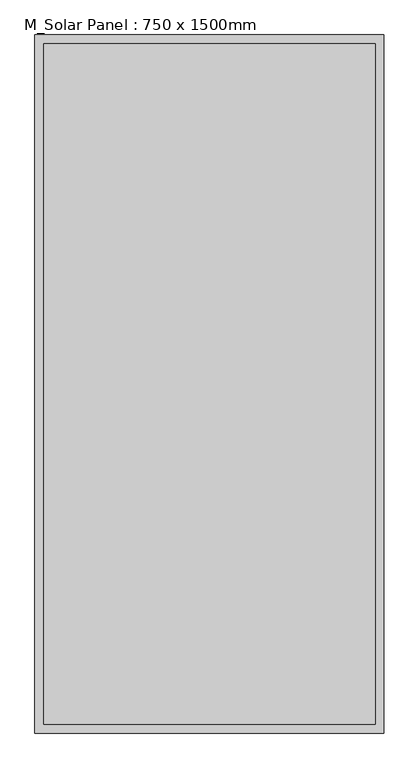
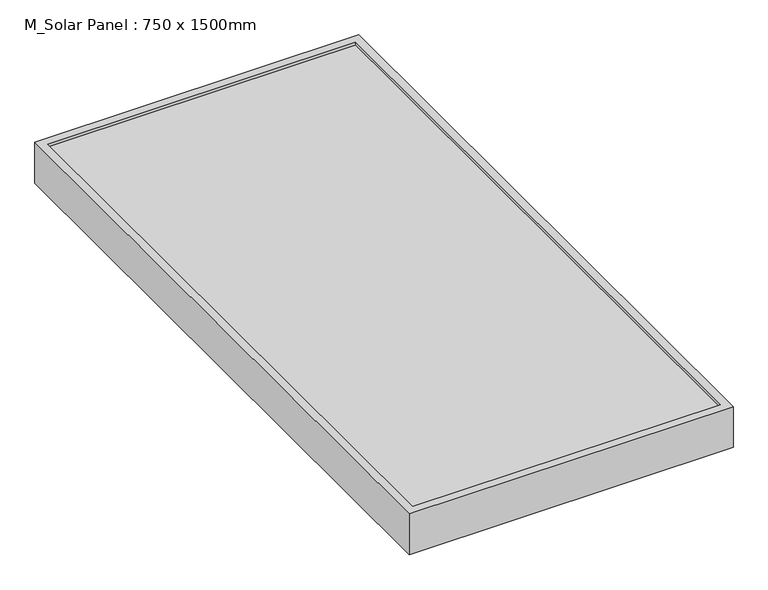
"""IFC4 building model written with IfcOpenShell, lengths in millimetres: proxy geometry, M_Solar Panel : 750 x 1500mm."""

from ifc_helpers import new_model, si_unit, origin, origin_with_axes, place, context, project, spatial, polyline, outline, extrude, source, transform, mapped, element, save


def m_solar_panel_750_x_1500mm_21fb4d5c(model_context):
    return source(origin(), model_context, "Body", "SweptSolid", [
        extrude(outline(polyline([(32.32, 1500.0), (782.32, 1500.0), (782.32, 0.0), (32.32, 0.0), (32.32, 1500.0)]), holes=[polyline([(763.27, 1480.95), (51.37, 1480.95), (51.37, 19.05), (763.27, 19.05), (763.27, 1480.95)])]), origin_with_axes(), (0.0, 0.0, 1.0), 100.0),
        extrude(outline(polyline([(763.27, 1480.95), (763.27, 19.05), (51.37, 19.05), (51.37, 1480.95), (763.27, 1480.95)])), origin_with_axes(), (0.0, 0.0, 1.0), 93.65),
    ])


if __name__ == "__main__":
    model = new_model("IFC4")
    model_context = context("Model", 3, world=origin())
    ifc_project = project(units=[si_unit("LENGTHUNIT", "METRE", prefix="MILLI")], contexts=[model_context])
    site = spatial("IfcSite", under=ifc_project)
    building = spatial("IfcBuilding", under=site)
    placement = place(None, origin())
    m_solar_panel_750_x_1500mm_shape = m_solar_panel_750_x_1500mm_21fb4d5c(model_context)
    element("IfcBuildingElementProxy", 1, Name="M_Solar Panel : 750 x 1500mm", ObjectType="M_Solar Panel : 750 x 1500mm", at=placement, inside=building, context=model_context, shape_type="MappedRepresentation", body=[
        mapped(m_solar_panel_750_x_1500mm_shape, transform((0.0, 0.0, 0.0), x_axis=(1.0, 0.0, 0.0), y_axis=(0.0, 1.0, 0.0), z_axis=(0.0, 0.0, 1.0))),
    ])
    save(model, "model.ifc")

# Revit data of these elements
# Type "M_Solar Panel : 750 x 1500mm"
#   Width = 0.75 m
#   Length = 1.5 m
#   Depth = 0.1 m
#   Default Elevation = 1.2 m
# Element 1 (IfcBuildingElementProxy, "M_Solar Panel : 750 x 1500mm")
#   Materials on its faces: "Metal Trim", "Metal - Aluminum (2)"
# Materials
#   "Metal Trim": class "Metal", colour RGB 247 247 247, transparency 0
#   "Metal - Aluminum (2)": class "Metal", colour RGB 247 247 247, transparency 0
